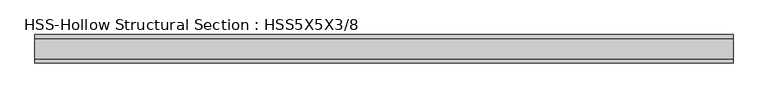
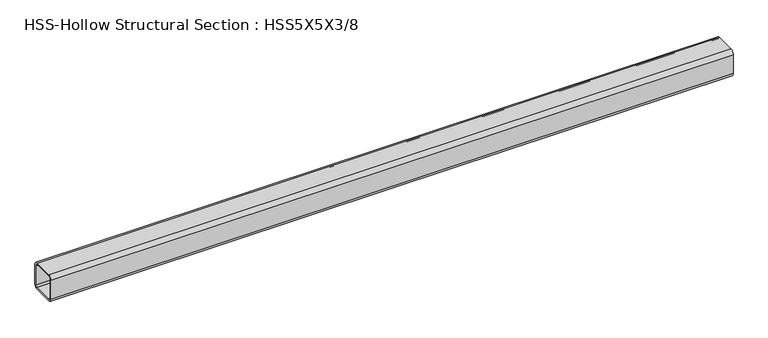
"""IFC4 building model written with IfcOpenShell, lengths in millimetres: member geometry, HSS-Hollow Structural Section : HSS5X5X3/8."""

from ifc_helpers import new_model, si_unit, point, frame, frame_2d, origin, place, context, project, spatial, polyline, circle_curve, trimmed, segment, composite_curve, outline, extrude, source, transform, mapped, element, save


def hss_hollow_structural_section_hss5x5x3_8_b689f2ae(model_context):
    return source(origin(), model_context, "Body", "SweptSolid", [
        extrude(outline(composite_curve([segment(polyline([(63.5, 45.7708), (63.5, -45.7708)]), True, "CONTINUOUS"), segment(trimmed(circle_curve(frame_2d((45.7708, -45.7708)), 17.7292), [point((63.5, -45.7708))], [point((45.7708, -63.5))], False, "CARTESIAN"), True, "CONTINUOUS"), segment(polyline([(45.7708, -63.5), (-45.7708, -63.5)]), True, "CONTINUOUS"), segment(trimmed(circle_curve(frame_2d((-45.7708, -45.7708)), 17.7292), [point((-45.7708, -63.5))], [point((-63.5, -45.7708))], False, "CARTESIAN"), True, "CONTINUOUS"), segment(polyline([(-63.5, -45.7708), (-63.5, 45.7708)]), True, "CONTINUOUS"), segment(trimmed(circle_curve(frame_2d((-45.7708, 45.7708)), 17.7292), [point((-63.5, 45.7708))], [point((-45.7708, 63.5))], False, "CARTESIAN"), True, "CONTINUOUS"), segment(polyline([(-45.7708, 63.5), (45.7708, 63.5)]), True, "CONTINUOUS"), segment(trimmed(circle_curve(frame_2d((45.7708, 45.7708)), 17.7292), [point((45.7708, 63.5))], [point((63.5, 45.7708))], False, "CARTESIAN"), True, "CONTINUOUS")], self_intersect=False), holes=[composite_curve([segment(trimmed(circle_curve(frame_2d((-45.7708, 45.7708)), 8.8646), [point((-45.7708, 54.6354))], [point((-54.6354, 45.7708))], True, "CARTESIAN"), True, "CONTINUOUS"), segment(polyline([(-54.6354, 45.7708), (-54.6354, -45.7708)]), True, "CONTINUOUS"), segment(trimmed(circle_curve(frame_2d((-45.7708, -45.7708)), 8.8646), [point((-54.6354, -45.7708))], [point((-45.7708, -54.6354))], True, "CARTESIAN"), True, "CONTINUOUS"), segment(polyline([(-45.7708, -54.6354), (45.7708, -54.6354)]), True, "CONTINUOUS"), segment(trimmed(circle_curve(frame_2d((45.7708, -45.7708)), 8.8646), [point((45.7708, -54.6354))], [point((54.6354, -45.7708))], True, "CARTESIAN"), True, "CONTINUOUS"), segment(polyline([(54.6354, -45.7708), (54.6354, 45.7708)]), True, "CONTINUOUS"), segment(trimmed(circle_curve(frame_2d((45.7708, 45.7708)), 8.8646), [point((54.6354, 45.7708))], [point((45.7708, 54.6354))], True, "CARTESIAN"), True, "CONTINUOUS"), segment(polyline([(45.7708, 54.6354), (-45.7708, 54.6354)]), True, "CONTINUOUS")], self_intersect=False)]), frame((-1539.5074524, 0.0, 0.0), z_axis=(1.0, 0.0, 0.0), x_axis=(0.0, 1.0, 0.0)), (0.0, 0.0, 1.0), 3114.5436004),
    ])


if __name__ == "__main__":
    model = new_model("IFC4")
    model_context = context("Model", 3, world=origin())
    ifc_project = project(units=[si_unit("LENGTHUNIT", "METRE", prefix="MILLI")], contexts=[model_context])
    site = spatial("IfcSite", under=ifc_project)
    building = spatial("IfcBuilding", under=site)
    placement = place(None, origin())
    hss_hollow_structural_section_hss5x5x3_8_shape = hss_hollow_structural_section_hss5x5x3_8_b689f2ae(model_context)
    element("IfcMember", 1, ObjectType="HSS-Hollow Structural Section : HSS5X5X3/8", at=placement, inside=building, context=model_context, shape_type="MappedRepresentation", body=[
        mapped(hss_hollow_structural_section_hss5x5x3_8_shape, transform((0.0, 0.0, 0.0), x_axis=(1.0, 0.0, 0.0), y_axis=(0.0, 1.0, 0.0), z_axis=(0.0, 0.0, 1.0))),
    ])
    save(model, "model.ifc")

# Revit data of these elements
# Type "HSS-Hollow Structural Section : HSS5X5X3/8"
#   Assembly Code = "B10"
#   Shape = "Square"
#   W = 22.3
#   Ht = 0' - 5"
#   Length [instance default] = 5' - 0"
#   b = 0' - 5"
#   kr = 0' - 0.698"
#   t = 0' - 0.349"
#   A = 0.0429167 SF
#   Structural Material [instance default] = Steel ASTM A500, Grade B, Rectangular and Square
# Element 1 (IfcMember, "HSS-Hollow Structural Section : HSS5X5X3/8")
#   Materials on its faces: "Steel ASTM A500, Grade B, Rectangular and Square"
# Materials
#   "Steel ASTM A500, Grade B, Rectangular and Square": class "Metal", colour RGB 199 199 199, transparency 0, Description = "Carbon steel", Cost = 0
